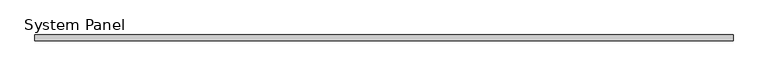
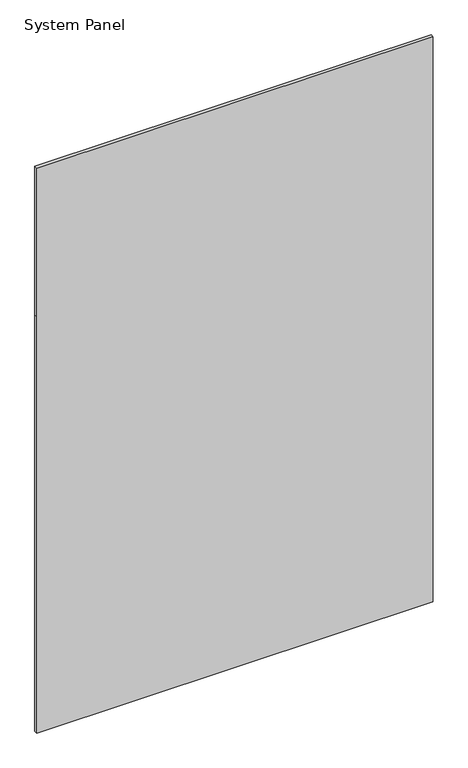
"""IFC4 building model written with IfcOpenShell, lengths in millimetres: plate geometry, System Panel : 로이복층유리_16."""

import ifcopenshell
import ifcopenshell.guid

model = None  # the IFC model being written
_history = None  # IfcOwnerHistory: only IFC2X3 demands one
_inside = {}  # id of a spatial element -> (the spatial element, [elements in it])
_under = {}  # id of a project, library or spatial element -> (it, [spatial elements below it])
_declared = {}  # id of a project -> (the project, [libraries it declares])
_typed = {}  # id of a type object -> (the type object, [elements of that type])
_made_of = {}  # id of a material, layer set ... -> (it, [elements and type objects made of it])


def new_model(schema):
    """Start an empty IFC model of exactly this schema.

    Asked for "IFC4X3", IfcOpenShell would pick the latest addendum, in which some entities
    have other attributes; the version numbers below select the first issue.
    IFC2X3 requires an IfcOwnerHistory on every rooted entity: one is made here for all.
    """
    global model, _history
    if schema == "IFC4X3":
        model = ifcopenshell.file(schema_version=(4, 3, 0, 0))
    else:
        model = ifcopenshell.file(schema=schema)
    _inside.clear()
    _under.clear()
    _declared.clear()
    _typed.clear()
    _made_of.clear()
    _history = None
    if model.schema == "IFC2X3":
        org = make("IfcOrganization", Name="unknown")
        user = make(
            "IfcPersonAndOrganization",
            ThePerson=make("IfcPerson", FamilyName="unknown"),
            TheOrganization=org,
        )
        app = make(
            "IfcApplication",
            ApplicationDeveloper=org,
            Version="unknown",
            ApplicationFullName="unknown",
            ApplicationIdentifier="unknown",
        )
        _history = make(
            "IfcOwnerHistory",
            OwningUser=user,
            OwningApplication=app,
            ChangeAction="ADDED",
            CreationDate=0,
        )
    return model


def make(cls, **values):
    """One entity of the class cls with the attributes given. An attribute that is None is left unset."""
    return model.create_entity(
        cls, **{name: value for name, value in values.items() if value is not None}
    )


def rooted(cls, **values):
    """An entity with a GlobalId (a new one), such as an element, a storey or a relation."""
    return make(cls, GlobalId=ifcopenshell.guid.new(), OwnerHistory=_history, **values)


def si_unit(unit_type, name, prefix=None):
    """IfcSIUnit, for example si_unit("LENGTHUNIT", "METRE", prefix="MILLI")."""
    return make("IfcSIUnit", UnitType=unit_type, Prefix=prefix, Name=name)


def assignment(units):
    """IfcUnitAssignment: the units of a project."""
    return None if units is None else make("IfcUnitAssignment", Units=units)


def point(xyz):
    """IfcCartesianPoint."""
    return None if xyz is None else make("IfcCartesianPoint", Coordinates=xyz)


def direction(xyz):
    """IfcDirection."""
    return None if xyz is None else make("IfcDirection", DirectionRatios=xyz)


def frame(location, z_axis=None, x_axis=None):
    """IfcAxis2Placement3D, a coordinate frame: its origin and axes. An axis left out is left unset."""
    return make(
        "IfcAxis2Placement3D",
        Location=point(location),
        Axis=direction(z_axis),
        RefDirection=direction(x_axis),
    )


def origin():
    """The frame at (0, 0, 0) with its axes left unset."""
    return frame((0.0, 0.0, 0.0))


def place(relative_to, where):
    """IfcLocalPlacement: puts the frame where relative to a parent placement (None: the world)."""
    return make(
        "IfcLocalPlacement", PlacementRelTo=relative_to, RelativePlacement=where
    )


def context(
    kind, dimensions, precision=None, world=None, true_north=None, identifier=None
):
    """IfcGeometricRepresentationContext, for example the 3D "Model" context."""
    return make(
        "IfcGeometricRepresentationContext",
        ContextIdentifier=identifier,
        ContextType=kind,
        CoordinateSpaceDimension=dimensions,
        Precision=precision,
        WorldCoordinateSystem=world,
        TrueNorth=true_north,
    )


def project(units=None, contexts=None):
    """IfcProject with its units and contexts."""
    return rooted(
        "IfcProject",
        Name="project",
        RepresentationContexts=contexts,
        UnitsInContext=assignment(units),
    )


def spatial(cls, under=None, at=None, **own):
    """A site, building, storey or space (cls), placed at a placement, below another one or the project."""
    s = rooted(cls, ObjectPlacement=at, **own)
    if under is not None:
        _under.setdefault(under.id(), (under, []))[1].append(s)
    return s


def polyline(points):
    """IfcPolyline through the points."""
    return make("IfcPolyline", Points=[point(p) for p in points])


def outline(outer, holes=None, kind="AREA"):
    """IfcArbitraryClosedProfileDef: a profile drawn as a closed curve; with holes, ...WithVoids."""
    if holes is None:
        return make("IfcArbitraryClosedProfileDef", ProfileType=kind, OuterCurve=outer)
    return make(
        "IfcArbitraryProfileDefWithVoids",
        ProfileType=kind,
        OuterCurve=outer,
        InnerCurves=holes,
    )


def extrude(swept, where, along, depth):
    """IfcExtrudedAreaSolid: the profile swept, set in the frame where, extruded along a direction by depth."""
    return make(
        "IfcExtrudedAreaSolid",
        SweptArea=swept,
        Position=where,
        ExtrudedDirection=direction(along),
        Depth=depth,
    )


def shape(context_of_items, identifier, shape_type, items):
    """IfcShapeRepresentation: the items that make up one representation, for example the "Body"."""
    return make(
        "IfcShapeRepresentation",
        ContextOfItems=context_of_items,
        RepresentationIdentifier=identifier,
        RepresentationType=shape_type,
        Items=items,
    )


def source(mapping_origin, context_of_items, identifier, shape_type, items):
    """IfcRepresentationMap: a shape defined once, which mapped items show again and again."""
    return make(
        "IfcRepresentationMap",
        MappingOrigin=mapping_origin,
        MappedRepresentation=shape(context_of_items, identifier, shape_type, items),
    )


def transform(
    local_origin,
    x_axis=None,
    y_axis=None,
    z_axis=None,
    scale=None,
    scale2=None,
    scale3=None,
    uniform=True,
):
    """IfcCartesianTransformationOperator3D, or its non-uniform kind. x_axis, y_axis, z_axis: its Axis1, 2, 3."""
    if uniform:
        return make(
            "IfcCartesianTransformationOperator3D",
            Axis1=direction(x_axis),
            Axis2=direction(y_axis),
            LocalOrigin=point(local_origin),
            Scale=scale,
            Axis3=direction(z_axis),
        )
    return make(
        "IfcCartesianTransformationOperator3DnonUniform",
        Axis1=direction(x_axis),
        Axis2=direction(y_axis),
        LocalOrigin=point(local_origin),
        Scale=scale,
        Axis3=direction(z_axis),
        Scale2=scale2,
        Scale3=scale3,
    )


def mapped(mapping_source, mapping_target):
    """IfcMappedItem: shows the shape of a source again, moved by a transform."""
    return make(
        "IfcMappedItem", MappingSource=mapping_source, MappingTarget=mapping_target
    )


def made_of(thing, what):
    """Note that an element or type object is made of a material, layer set ...; save() writes the relation."""
    if what is not None:
        _made_of.setdefault(what.id(), (what, []))[1].append(thing)
    return thing


def element(
    cls,
    number,
    at=None,
    inside=None,
    cuts=None,
    type_object=None,
    material=None,
    context=None,
    identifier="Body",
    shape_type=None,
    held_by="IfcProductDefinitionShape",
    body=None,
    shapes=None,
    **own,
):
    """One element of the class cls, such as IfcWall. Its Tag is "e" and its number.

    at: its placement. inside: the storey or other place that contains it. cuts: it is an
    opening in that element (IfcRelVoidsElement). A single representation is given by context,
    identifier, shape_type and body (its items); several are given by shapes. held_by: the class
    of the entity that holds the representations. save() writes the other relations.
    """
    e = rooted(cls, Tag="e%d" % number, ObjectPlacement=at, **own)
    if body is not None:
        shapes = [shape(context, identifier, shape_type, body)]
    if shapes is not None:
        e.Representation = make(held_by, Representations=shapes)
    if inside is not None:
        _inside.setdefault(inside.id(), (inside, []))[1].append(e)
    if cuts is not None:
        rooted(
            "IfcRelVoidsElement", RelatingBuildingElement=cuts, RelatedOpeningElement=e
        )
    if type_object is not None:
        _typed.setdefault(type_object.id(), (type_object, []))[1].append(e)
    return made_of(e, material)


def aggregate(whole, parts):
    """IfcRelAggregates: a whole, such as a stair, and the parts it consists of."""
    return rooted("IfcRelAggregates", RelatingObject=whole, RelatedObjects=parts)


def save(model, path):
    """Write the relations noted so far, then the file.

    IfcRelAggregates (storeys below a building ...), IfcRelContainedInSpatialStructure (elements
    in a storey), IfcRelDefinesByType, IfcRelAssociatesMaterial and IfcRelDeclares: one each for
    every whole, place, type object, material and project.
    """
    for whole, parts in _under.values():
        aggregate(whole, parts)
    for where, things in _inside.values():
        rooted(
            "IfcRelContainedInSpatialStructure",
            RelatedElements=things,
            RelatingStructure=where,
        )
    for kind, things in _typed.values():
        rooted("IfcRelDefinesByType", RelatedObjects=things, RelatingType=kind)
    for what, things in _made_of.values():
        rooted("IfcRelAssociatesMaterial", RelatedObjects=things, RelatingMaterial=what)
    for by, libraries in _declared.values():
        rooted("IfcRelDeclares", RelatingContext=by, RelatedDefinitions=libraries)
    model.write(path)


def system_panel_778a0f69(model_context):
    return source(origin(), model_context, "Body", "SweptSolid", [
        extrude(outline(polyline([(0.0, -980.9999999), (0.0, 980.9999999), (2177.5, 980.9999999), (2955.0, 980.9999999), (2955.0, -980.9999999), (2177.5, -980.9999999), (0.0, -980.9999999)])), frame((0.0, -8.0, 0.0), z_axis=(0.0, 1.0, 0.0), x_axis=(0.0, 0.0, 1.0)), (0.0, 0.0, 1.0), 16.0),
    ])


if __name__ == "__main__":
    model = new_model("IFC4")
    model_context = context("Model", 3, world=origin())
    ifc_project = project(units=[si_unit("LENGTHUNIT", "METRE", prefix="MILLI")], contexts=[model_context])
    site = spatial("IfcSite", under=ifc_project)
    building = spatial("IfcBuilding", under=site)
    placement = place(None, origin())
    system_panel_shape = system_panel_778a0f69(model_context)
    element("IfcPlate", 1, ObjectType="System Panel : 로이복층유리_16", at=placement, inside=building, context=model_context, shape_type="MappedRepresentation", body=[
        mapped(system_panel_shape, transform((0.0, 0.0, 0.0), x_axis=(1.0, 0.0, 0.0), y_axis=(0.0, 1.0, 0.0), z_axis=(0.0, 0.0, 1.0))),
    ])
    save(model, "model.ifc")

# Revit data of these elements
# Element 1 (IfcPlate, "System Panel : 로이복층유리_16")
#   Materials on its faces: "00_Glass_Glass"
# Materials
#   "00_Glass_Glass": class "Glass", colour RGB 218 227 224, transparency 0.85, Description = "Glass", Cost = 0, Image = none
